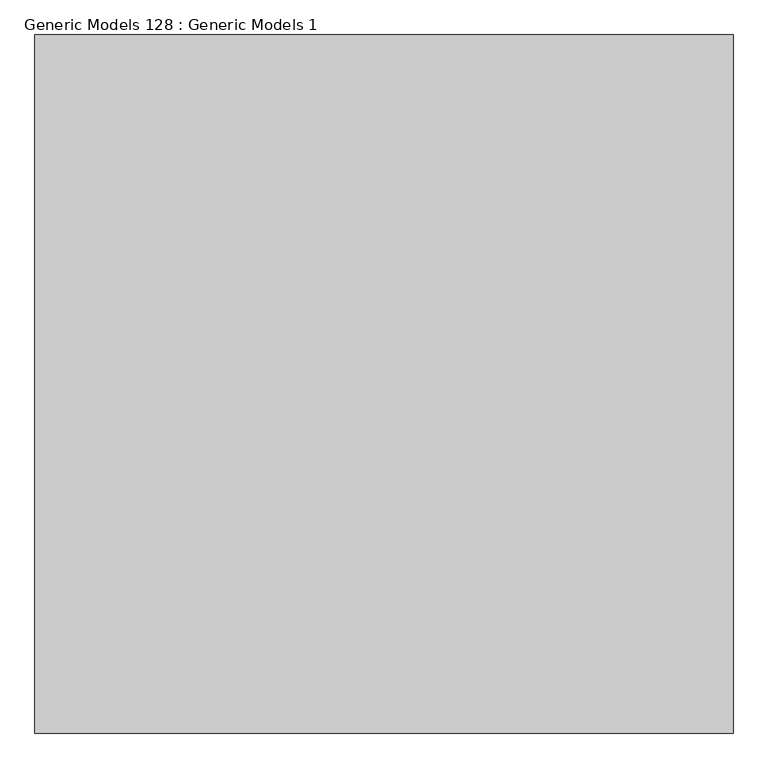
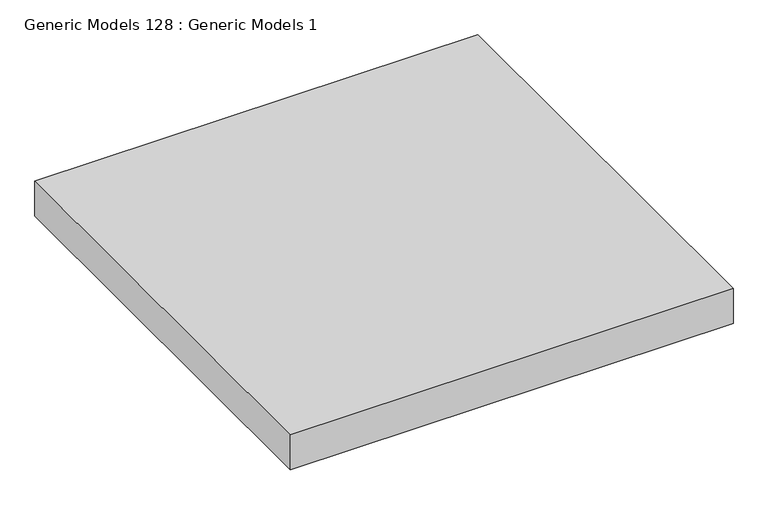
"""IFC4 building model written with IfcOpenShell, lengths in millimetres: proxy geometry, Generic Models 128 : Generic Models 1."""

import ifcopenshell
import ifcopenshell.guid

model = None  # the IFC model being written
_history = None  # IfcOwnerHistory: only IFC2X3 demands one
_inside = {}  # id of a spatial element -> (the spatial element, [elements in it])
_under = {}  # id of a project, library or spatial element -> (it, [spatial elements below it])
_declared = {}  # id of a project -> (the project, [libraries it declares])
_typed = {}  # id of a type object -> (the type object, [elements of that type])
_made_of = {}  # id of a material, layer set ... -> (it, [elements and type objects made of it])


def new_model(schema):
    """Start an empty IFC model of exactly this schema.

    Asked for "IFC4X3", IfcOpenShell would pick the latest addendum, in which some entities
    have other attributes; the version numbers below select the first issue.
    IFC2X3 requires an IfcOwnerHistory on every rooted entity: one is made here for all.
    """
    global model, _history
    if schema == "IFC4X3":
        model = ifcopenshell.file(schema_version=(4, 3, 0, 0))
    else:
        model = ifcopenshell.file(schema=schema)
    _inside.clear()
    _under.clear()
    _declared.clear()
    _typed.clear()
    _made_of.clear()
    _history = None
    if model.schema == "IFC2X3":
        org = make("IfcOrganization", Name="unknown")
        user = make(
            "IfcPersonAndOrganization",
            ThePerson=make("IfcPerson", FamilyName="unknown"),
            TheOrganization=org,
        )
        app = make(
            "IfcApplication",
            ApplicationDeveloper=org,
            Version="unknown",
            ApplicationFullName="unknown",
            ApplicationIdentifier="unknown",
        )
        _history = make(
            "IfcOwnerHistory",
            OwningUser=user,
            OwningApplication=app,
            ChangeAction="ADDED",
            CreationDate=0,
        )
    return model


def make(cls, **values):
    """One entity of the class cls with the attributes given. An attribute that is None is left unset."""
    return model.create_entity(
        cls, **{name: value for name, value in values.items() if value is not None}
    )


def rooted(cls, **values):
    """An entity with a GlobalId (a new one), such as an element, a storey or a relation."""
    return make(cls, GlobalId=ifcopenshell.guid.new(), OwnerHistory=_history, **values)


def si_unit(unit_type, name, prefix=None):
    """IfcSIUnit, for example si_unit("LENGTHUNIT", "METRE", prefix="MILLI")."""
    return make("IfcSIUnit", UnitType=unit_type, Prefix=prefix, Name=name)


def assignment(units):
    """IfcUnitAssignment: the units of a project."""
    return None if units is None else make("IfcUnitAssignment", Units=units)


def point(xyz):
    """IfcCartesianPoint."""
    return None if xyz is None else make("IfcCartesianPoint", Coordinates=xyz)


def direction(xyz):
    """IfcDirection."""
    return None if xyz is None else make("IfcDirection", DirectionRatios=xyz)


def frame(location, z_axis=None, x_axis=None):
    """IfcAxis2Placement3D, a coordinate frame: its origin and axes. An axis left out is left unset."""
    return make(
        "IfcAxis2Placement3D",
        Location=point(location),
        Axis=direction(z_axis),
        RefDirection=direction(x_axis),
    )


def origin():
    """The frame at (0, 0, 0) with its axes left unset."""
    return frame((0.0, 0.0, 0.0))


def place(relative_to, where):
    """IfcLocalPlacement: puts the frame where relative to a parent placement (None: the world)."""
    return make(
        "IfcLocalPlacement", PlacementRelTo=relative_to, RelativePlacement=where
    )


def context(
    kind, dimensions, precision=None, world=None, true_north=None, identifier=None
):
    """IfcGeometricRepresentationContext, for example the 3D "Model" context."""
    return make(
        "IfcGeometricRepresentationContext",
        ContextIdentifier=identifier,
        ContextType=kind,
        CoordinateSpaceDimension=dimensions,
        Precision=precision,
        WorldCoordinateSystem=world,
        TrueNorth=true_north,
    )


def project(units=None, contexts=None):
    """IfcProject with its units and contexts."""
    return rooted(
        "IfcProject",
        Name="project",
        RepresentationContexts=contexts,
        UnitsInContext=assignment(units),
    )


def spatial(cls, under=None, at=None, **own):
    """A site, building, storey or space (cls), placed at a placement, below another one or the project."""
    s = rooted(cls, ObjectPlacement=at, **own)
    if under is not None:
        _under.setdefault(under.id(), (under, []))[1].append(s)
    return s


def polyline(points):
    """IfcPolyline through the points."""
    return make("IfcPolyline", Points=[point(p) for p in points])


def outline(outer, holes=None, kind="AREA"):
    """IfcArbitraryClosedProfileDef: a profile drawn as a closed curve; with holes, ...WithVoids."""
    if holes is None:
        return make("IfcArbitraryClosedProfileDef", ProfileType=kind, OuterCurve=outer)
    return make(
        "IfcArbitraryProfileDefWithVoids",
        ProfileType=kind,
        OuterCurve=outer,
        InnerCurves=holes,
    )


def extrude(swept, where, along, depth):
    """IfcExtrudedAreaSolid: the profile swept, set in the frame where, extruded along a direction by depth."""
    return make(
        "IfcExtrudedAreaSolid",
        SweptArea=swept,
        Position=where,
        ExtrudedDirection=direction(along),
        Depth=depth,
    )


def shape(context_of_items, identifier, shape_type, items):
    """IfcShapeRepresentation: the items that make up one representation, for example the "Body"."""
    return make(
        "IfcShapeRepresentation",
        ContextOfItems=context_of_items,
        RepresentationIdentifier=identifier,
        RepresentationType=shape_type,
        Items=items,
    )


def source(mapping_origin, context_of_items, identifier, shape_type, items):
    """IfcRepresentationMap: a shape defined once, which mapped items show again and again."""
    return make(
        "IfcRepresentationMap",
        MappingOrigin=mapping_origin,
        MappedRepresentation=shape(context_of_items, identifier, shape_type, items),
    )


def transform(
    local_origin,
    x_axis=None,
    y_axis=None,
    z_axis=None,
    scale=None,
    scale2=None,
    scale3=None,
    uniform=True,
):
    """IfcCartesianTransformationOperator3D, or its non-uniform kind. x_axis, y_axis, z_axis: its Axis1, 2, 3."""
    if uniform:
        return make(
            "IfcCartesianTransformationOperator3D",
            Axis1=direction(x_axis),
            Axis2=direction(y_axis),
            LocalOrigin=point(local_origin),
            Scale=scale,
            Axis3=direction(z_axis),
        )
    return make(
        "IfcCartesianTransformationOperator3DnonUniform",
        Axis1=direction(x_axis),
        Axis2=direction(y_axis),
        LocalOrigin=point(local_origin),
        Scale=scale,
        Axis3=direction(z_axis),
        Scale2=scale2,
        Scale3=scale3,
    )


def mapped(mapping_source, mapping_target):
    """IfcMappedItem: shows the shape of a source again, moved by a transform."""
    return make(
        "IfcMappedItem", MappingSource=mapping_source, MappingTarget=mapping_target
    )


def made_of(thing, what):
    """Note that an element or type object is made of a material, layer set ...; save() writes the relation."""
    if what is not None:
        _made_of.setdefault(what.id(), (what, []))[1].append(thing)
    return thing


def element(
    cls,
    number,
    at=None,
    inside=None,
    cuts=None,
    type_object=None,
    material=None,
    context=None,
    identifier="Body",
    shape_type=None,
    held_by="IfcProductDefinitionShape",
    body=None,
    shapes=None,
    **own,
):
    """One element of the class cls, such as IfcWall. Its Tag is "e" and its number.

    at: its placement. inside: the storey or other place that contains it. cuts: it is an
    opening in that element (IfcRelVoidsElement). A single representation is given by context,
    identifier, shape_type and body (its items); several are given by shapes. held_by: the class
    of the entity that holds the representations. save() writes the other relations.
    """
    e = rooted(cls, Tag="e%d" % number, ObjectPlacement=at, **own)
    if body is not None:
        shapes = [shape(context, identifier, shape_type, body)]
    if shapes is not None:
        e.Representation = make(held_by, Representations=shapes)
    if inside is not None:
        _inside.setdefault(inside.id(), (inside, []))[1].append(e)
    if cuts is not None:
        rooted(
            "IfcRelVoidsElement", RelatingBuildingElement=cuts, RelatedOpeningElement=e
        )
    if type_object is not None:
        _typed.setdefault(type_object.id(), (type_object, []))[1].append(e)
    return made_of(e, material)


def aggregate(whole, parts):
    """IfcRelAggregates: a whole, such as a stair, and the parts it consists of."""
    return rooted("IfcRelAggregates", RelatingObject=whole, RelatedObjects=parts)


def save(model, path):
    """Write the relations noted so far, then the file.

    IfcRelAggregates (storeys below a building ...), IfcRelContainedInSpatialStructure (elements
    in a storey), IfcRelDefinesByType, IfcRelAssociatesMaterial and IfcRelDeclares: one each for
    every whole, place, type object, material and project.
    """
    for whole, parts in _under.values():
        aggregate(whole, parts)
    for where, things in _inside.values():
        rooted(
            "IfcRelContainedInSpatialStructure",
            RelatedElements=things,
            RelatingStructure=where,
        )
    for kind, things in _typed.values():
        rooted("IfcRelDefinesByType", RelatedObjects=things, RelatingType=kind)
    for what, things in _made_of.values():
        rooted("IfcRelAssociatesMaterial", RelatedObjects=things, RelatingMaterial=what)
    for by, libraries in _declared.values():
        rooted("IfcRelDeclares", RelatingContext=by, RelatedDefinitions=libraries)
    model.write(path)


def generic_models_128_generic_models_1_9921986f(model_context):
    return source(origin(), model_context, "Body", "SweptSolid", [
        extrude(outline(polyline([(47499.4360531, 0.0), (46280.2360531, 0.0), (46280.2360531, 1219.2), (47499.4360531, 1219.2), (47499.4360531, 0.0)])), frame((0.0, 0.0, 2231.473933), z_axis=(0.0, 0.0, 1.0), x_axis=(1.0, 0.0, 0.0)), (0.0, 0.0, 1.0), 101.6),
    ])


if __name__ == "__main__":
    model = new_model("IFC4")
    model_context = context("Model", 3, world=origin())
    ifc_project = project(units=[si_unit("LENGTHUNIT", "METRE", prefix="MILLI")], contexts=[model_context])
    site = spatial("IfcSite", under=ifc_project)
    building = spatial("IfcBuilding", under=site)
    placement = place(None, origin())
    generic_models_128_generic_models_1_shape = generic_models_128_generic_models_1_9921986f(model_context)
    element("IfcBuildingElementProxy", 1, Name="Generic Models 128 : Generic Models 1", ObjectType="Generic Models 128 : Generic Models 1", at=placement, inside=building, context=model_context, shape_type="MappedRepresentation", body=[
        mapped(generic_models_128_generic_models_1_shape, transform((0.0, 0.0, 0.0), x_axis=(1.0, 0.0, 0.0), y_axis=(0.0, 1.0, 0.0), z_axis=(0.0, 0.0, 1.0))),
    ])
    save(model, "model.ifc")

# Revit data of these elements
# Element 1 (IfcBuildingElementProxy, "Generic Models 128 : Generic Models 1")
#   Materials on its faces: "UNDERSIDE OF STRUCTURE"
# Materials
#   "UNDERSIDE OF STRUCTURE": class "Concrete", colour RGB 129 132 118, transparency 0, Description = "Lightweight concrete", Cost = 0
